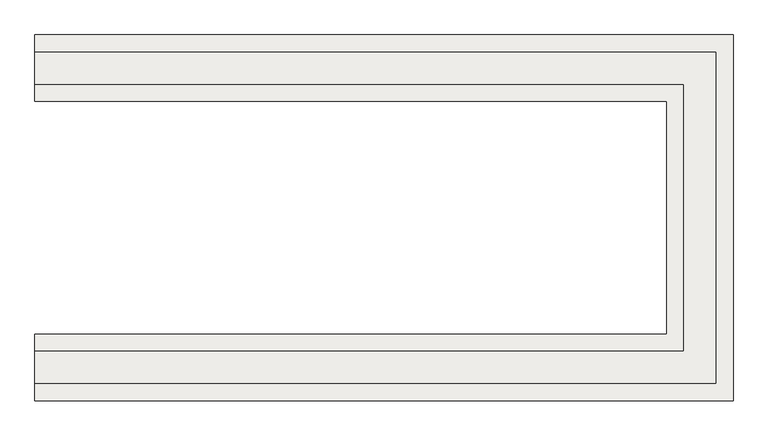
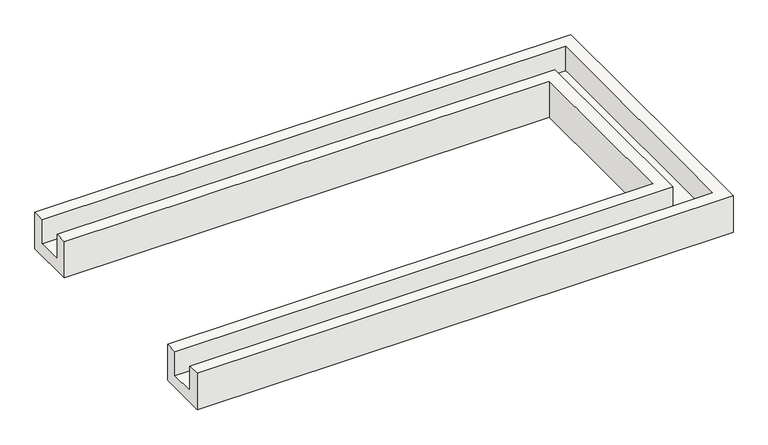
"""IFC4 building model written with IfcOpenShell, lengths in millimetres: slab geometry, 구조 기초 1 : 구조 기초 1."""

from ifc_helpers import new_model, si_unit, origin, place, context, project, spatial, faceted_brep, source, transform, mapped, element, save


def slab_6818e2bc(model_context):
    return source(origin(), model_context, "Body", "Brep", [
        faceted_brep([(-7160.8345066, 14987.9196162, 599.9720055), (-7160.8345066, 15237.9196162, 599.9720055), (-7160.8345066, 15237.9196162, 99.9720055), (-7160.8345066, 15737.9196162, 99.9720055), (-7160.8345066, 15737.9196162, 599.9720055), (-7160.8345066, 15987.9196162, 599.9720055), (-7160.8345066, 15987.9196162, -150.0279945), (-7160.8345066, 14987.9196162, -150.0279945), (3339.1654934, 15987.9196162, -150.0279945), (3339.1654934, 10487.9196162, -150.0279945), (-7160.8345066, 10487.9196162, -150.0279945), (-7160.8345066, 11487.9196162, -150.0279945), (2339.1654934, 11487.9196162, -150.0279945), (2339.1654934, 14987.9196162, -150.0279945), (2339.1654934, 14987.9196162, 599.9720055), (2339.1654934, 11487.9196162, 599.9720055), (-7160.8345066, 11487.9196162, 599.9720055), (-7160.8345066, 11237.9196162, 599.9720055), (2589.1654934, 11237.9196162, 599.9720055), (2589.1654934, 15237.9196162, 599.9720055), (2589.1654934, 15237.9196162, 99.9720055), (2589.1654934, 11237.9196162, 99.9720055), (-7160.8345066, 10487.9196162, 599.9720055), (-7160.8345066, 10737.9196162, 599.9720055), (-7160.8345066, 10737.9196162, 99.9720055), (-7160.8345066, 11237.9196162, 99.9720055), (3089.1654934, 10737.9196162, 99.9720055), (3089.1654934, 15737.9196162, 99.9720055), (3089.1654934, 15737.9196162, 599.9720055), (3089.1654934, 10737.9196162, 599.9720055), (3339.1654934, 10487.9196162, 599.9720055), (3339.1654934, 15987.9196162, 599.9720055)], [[[0, 1, 2, 3, 4, 5, 6, 7]], [[6, 8, 9, 10, 11, 12, 13, 7]], [[0, 7, 13, 14]], [[1, 0, 14, 15, 16, 17, 18, 19]], [[2, 1, 19, 20]], [[14, 13, 12, 15]], [[20, 19, 18, 21]], [[16, 11, 10, 22, 23, 24, 25, 17]], [[15, 12, 11, 16]], [[21, 18, 17, 25]], [[2, 20, 21, 25, 24, 26, 27, 3]], [[4, 3, 27, 28]], [[5, 4, 28, 29, 23, 22, 30, 31]], [[6, 5, 31, 8]], [[28, 27, 26, 29]], [[8, 31, 30, 9]], [[29, 26, 24, 23]], [[9, 30, 22, 10]]]),
    ])


if __name__ == "__main__":
    model = new_model("IFC4")
    model_context = context("Model", 3, world=origin())
    ifc_project = project(units=[si_unit("LENGTHUNIT", "METRE", prefix="MILLI")], contexts=[model_context])
    site = spatial("IfcSite", under=ifc_project)
    building = spatial("IfcBuilding", under=site)
    placement = place(None, origin())
    slab_shape = slab_6818e2bc(model_context)
    element("IfcSlab", 1, ObjectType="구조 기초 1 : 구조 기초 1", at=placement, inside=building, context=model_context, shape_type="MappedRepresentation", body=[
        mapped(slab_shape, transform((0.0, 0.0, 0.0), x_axis=(1.0, 0.0, 0.0), y_axis=(0.0, 1.0, 0.0), z_axis=(0.0, 0.0, 1.0))),
    ])
    save(model, "model.ifc")

# Revit data of these elements
# Type "구조 기초 1 : 구조 기초 1"
#   Volume [instance default] = 12.2500 m
#   THeight [instance default] = 0.7500 m
#   T2Length [instance default] = 5.5000 m
#   T1Width [instance default] = 1.0000 m
#   T1Length [instance default] = 9.5000 m
#   DHeight [instance default] = 0.5000 m
#   D2Width [instance default] = 0.2500 m
#   D1Width [instance default] = 0.5000 m
